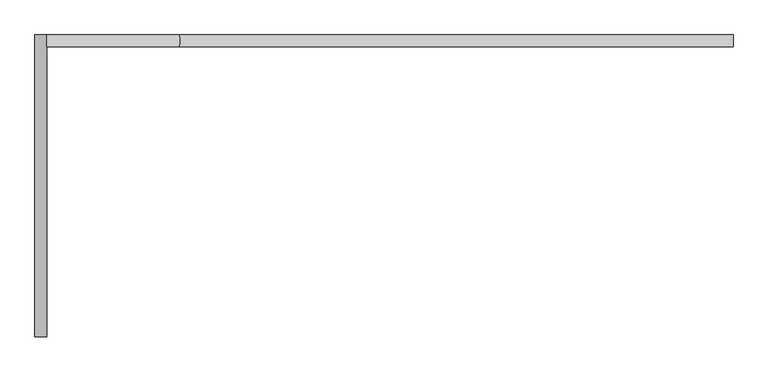
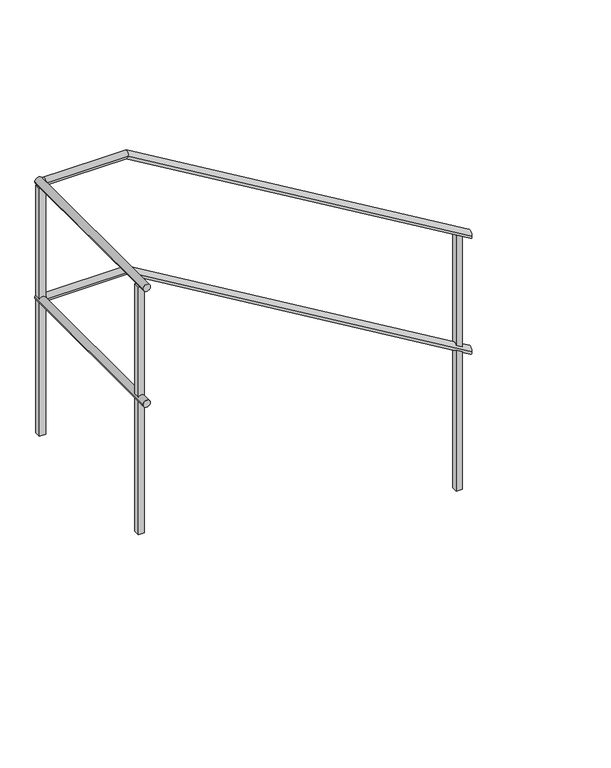
"""IFC4 building model written with IfcOpenShell, lengths in millimetres: railing geometry."""

from ifc_helpers import new_model, si_unit, frame, origin, place, context, project, spatial, polyline, circle_curve, ellipse_curve, outline, extrude, source, transform, mapped, element, save
from ifc_brep_helpers import plane_surface, cylinder_surface, advanced_brep


def railing_e85a09c7(model_context):
    return source(origin(), model_context, "Body", "SolidModel", [
        advanced_brep(
        [(33043.8956602, 24484.5208589, 749.1723166), (33043.8956602, 24514.5208589, 749.1723166), (31639.7692216, 24484.5208589, 1584.9618634), (31639.7692216, 24514.5208589, 1584.9618634), (31305.4, 24484.5208589, 1584.9618634), (31305.4, 24514.5208589, 1584.9618634)],
        [
            (0, 1, ellipse_curve(frame((33043.8956602, 24499.5208589, 749.1723166), z_axis=(1.0, 0.0, 0.0), x_axis=(0.0, 0.0, -1.0)), 17.4562134, 15.0)),
            (1, 0, ellipse_curve(frame((33043.8956602, 24499.5208589, 749.1723166), z_axis=(1.0, 0.0, 0.0), x_axis=(0.0, 0.0, -1.0)), 17.4562134, 15.0)),
            (0, 2),
            (2, 3, ellipse_curve(frame((31639.7692216, 24499.5208589, 1584.9618634), z_axis=(0.9641817474962141, 0.0, -0.2652424509673118), x_axis=(-0.265242450967312, 0.0, -0.9641817474962139)), 15.5572329, 15.0)),
            (3, 1),
            (3, 2, ellipse_curve(frame((31639.7692216, 24499.5208589, 1584.9618634), z_axis=(0.9641817474962141, 0.0, -0.2652424509673118), x_axis=(-0.265242450967312, 0.0, -0.9641817474962139)), 15.5572329, 15.0)),
            (4, 5, circle_curve(frame((31305.4, 24499.5208589, 1584.9618634), z_axis=(-1.0, 0.0, 0.0), x_axis=(0.0, 1.0, 0.0)), 15.0)),
            (5, 4, circle_curve(frame((31305.4, 24499.5208589, 1584.9618634), z_axis=(-1.0, 0.0, 0.0), x_axis=(0.0, 1.0, 0.0)), 15.0)),
            (2, 4),
            (5, 3),
        ],
        [
            plane_surface(frame((33043.8956602, 24499.5208589, 766.62853), z_axis=(1.0, 0.0, 0.0), x_axis=(0.0, -1.0, 0.0))),
            cylinder_surface(frame((33036.2234023, 24499.5208589, 753.7391368), z_axis=(0.8592928844097064, 0.0, -0.5114838597676831), x_axis=(0.0, 1.0, 0.0)), 15.0),
            plane_surface(frame((31305.4, 24499.5208589, 1599.9618634), z_axis=(-1.0, 0.0, 0.0), x_axis=(0.0, -1.0, 0.0))),
            cylinder_surface(frame((31643.8956602, 24499.5208589, 1584.9618634), z_axis=(1.0, 0.0, 0.0), x_axis=(0.0, 1.0, 0.0)), 15.0),
        ],
        [
            (0, [[1, 2]]),
            (1, [[-1, 3, 4, 5]]),
            (1, [[-2, -5, 6, -3]]),
            (2, [[7, 8]]),
            (3, [[-4, 9, -8, 10]]),
            (3, [[-6, -10, -7, -9]]),
        ],
    ),
        advanced_brep(
        [(33043.8956602, 24484.5208589, 1249.1723166), (33043.8956602, 24514.5208589, 1249.1723166), (31639.7692216, 24484.5208589, 2084.9618634), (31639.7692216, 24514.5208589, 2084.9618634), (31305.4, 24484.5208589, 2084.9618634), (31305.4, 24514.5208589, 2084.9618634)],
        [
            (0, 1, ellipse_curve(frame((33043.8956602, 24499.5208589, 1249.1723166), z_axis=(1.0, 0.0, 0.0), x_axis=(0.0, 0.0, -1.0)), 17.4562134, 15.0)),
            (1, 0, ellipse_curve(frame((33043.8956602, 24499.5208589, 1249.1723166), z_axis=(1.0, 0.0, 0.0), x_axis=(0.0, 0.0, -1.0)), 17.4562134, 15.0)),
            (0, 2),
            (2, 3, ellipse_curve(frame((31639.7692216, 24499.5208589, 2084.9618634), z_axis=(0.9641817474962141, 0.0, -0.2652424509673118), x_axis=(-0.265242450967312, 0.0, -0.9641817474962139)), 15.5572329, 15.0)),
            (3, 1),
            (3, 2, ellipse_curve(frame((31639.7692216, 24499.5208589, 2084.9618634), z_axis=(0.9641817474962141, 0.0, -0.2652424509673118), x_axis=(-0.265242450967312, 0.0, -0.9641817474962139)), 15.5572329, 15.0)),
            (4, 5, circle_curve(frame((31305.4, 24499.5208589, 2084.9618634), z_axis=(-1.0, 0.0, 0.0), x_axis=(0.0, 1.0, 0.0)), 15.0)),
            (5, 4, circle_curve(frame((31305.4, 24499.5208589, 2084.9618634), z_axis=(-1.0, 0.0, 0.0), x_axis=(0.0, 1.0, 0.0)), 15.0)),
            (2, 4),
            (5, 3),
        ],
        [
            plane_surface(frame((33043.8956602, 24499.5208589, 1266.62853), z_axis=(1.0, 0.0, 0.0), x_axis=(0.0, -1.0, 0.0))),
            cylinder_surface(frame((33036.2234023, 24499.5208589, 1253.7391368), z_axis=(0.8592928844097064, 0.0, -0.5114838597676831), x_axis=(0.0, 1.0, 0.0)), 15.0),
            plane_surface(frame((31305.4, 24499.5208589, 2099.9618634), z_axis=(-1.0, 0.0, 0.0), x_axis=(0.0, -1.0, 0.0))),
            cylinder_surface(frame((31643.8956602, 24499.5208589, 2084.9618634), z_axis=(1.0, 0.0, 0.0), x_axis=(0.0, 1.0, 0.0)), 15.0),
        ],
        [
            (0, [[1, 2]]),
            (1, [[-1, 3, 4, 5]]),
            (1, [[-2, -5, 6, -3]]),
            (2, [[7, 8]]),
            (3, [[-4, 9, -8, 10]]),
            (3, [[-6, -10, -7, -9]]),
        ],
    ),
        advanced_brep(
        [(31305.4, 24514.5208589, 1584.9618634), (31275.4, 24514.5208589, 1584.9618634), (31305.4, 23749.5208589, 1584.9618634), (31275.4, 23749.5208589, 1584.9618634)],
        [
            (0, 1, circle_curve(frame((31290.4, 24514.5208589, 1584.9618634), z_axis=(0.0, 1.0, 0.0), x_axis=(-1.0, 0.0, 0.0)), 15.0)),
            (1, 0, circle_curve(frame((31290.4, 24514.5208589, 1584.9618634), z_axis=(0.0, 1.0, 0.0), x_axis=(-1.0, 0.0, 0.0)), 15.0)),
            (2, 3, circle_curve(frame((31290.4, 23749.5208589, 1584.9618634), z_axis=(0.0, -1.0, 0.0), x_axis=(-1.0, 0.0, 0.0)), 15.0)),
            (3, 2, circle_curve(frame((31290.4, 23749.5208589, 1584.9618634), z_axis=(0.0, -1.0, 0.0), x_axis=(-1.0, 0.0, 0.0)), 15.0)),
            (0, 2),
            (3, 1),
        ],
        [
            plane_surface(frame((31290.4, 24514.5208589, 1599.9618634), z_axis=(0.0, 1.0, 0.0), x_axis=(0.0, 0.0, -1.0))),
            plane_surface(frame((31290.4, 23749.5208589, 1599.9618634), z_axis=(0.0, -1.0, 0.0), x_axis=(0.0, 0.0, -1.0))),
            cylinder_surface(frame((31290.4, 24514.5208589, 1584.9618634), z_axis=(0.0, 1.0, 0.0), x_axis=(-1.0, 0.0, 0.0)), 15.0),
        ],
        [
            (0, [[1, 2]]),
            (1, [[3, 4]]),
            (2, [[-1, 5, -4, 6]]),
            (2, [[-2, -6, -3, -5]]),
        ],
    ),
        advanced_brep(
        [(31305.4, 24514.5208589, 2084.9618634), (31275.4, 24514.5208589, 2084.9618634), (31305.4, 23749.5208589, 2084.9618634), (31275.4, 23749.5208589, 2084.9618634)],
        [
            (0, 1, circle_curve(frame((31290.4, 24514.5208589, 2084.9618634), z_axis=(0.0, 1.0, 0.0), x_axis=(-1.0, 0.0, 0.0)), 15.0)),
            (1, 0, circle_curve(frame((31290.4, 24514.5208589, 2084.9618634), z_axis=(0.0, 1.0, 0.0), x_axis=(-1.0, 0.0, 0.0)), 15.0)),
            (2, 3, circle_curve(frame((31290.4, 23749.5208589, 2084.9618634), z_axis=(0.0, -1.0, 0.0), x_axis=(-1.0, 0.0, 0.0)), 15.0)),
            (3, 2, circle_curve(frame((31290.4, 23749.5208589, 2084.9618634), z_axis=(0.0, -1.0, 0.0), x_axis=(-1.0, 0.0, 0.0)), 15.0)),
            (0, 2),
            (3, 1),
        ],
        [
            plane_surface(frame((31290.4, 24514.5208589, 2099.9618634), z_axis=(0.0, 1.0, 0.0), x_axis=(0.0, 0.0, -1.0))),
            plane_surface(frame((31290.4, 23749.5208589, 2099.9618634), z_axis=(0.0, -1.0, 0.0), x_axis=(0.0, 0.0, -1.0))),
            cylinder_surface(frame((31290.4, 24514.5208589, 2084.9618634), z_axis=(0.0, 1.0, 0.0), x_axis=(-1.0, 0.0, 0.0)), 15.0),
        ],
        [
            (0, [[1, 2]]),
            (1, [[3, 4]]),
            (2, [[-1, 5, -4, 6]]),
            (2, [[-2, -6, -3, -5]]),
        ],
    ),
        extrude(outline(polyline([(31302.9, 24512.0208589), (31302.9, 24487.0208589), (31277.9, 24487.0208589), (31277.9, 24512.0208589), (31302.9, 24512.0208589)])), frame((0.0, 0.0, 999.9618634), z_axis=(0.0, 0.0, 1.0), x_axis=(1.0, 0.0, 0.0)), (0.0, 0.0, 1.0), 1070.0),
        extrude(outline(polyline([(31277.9, 23812.0208589), (31302.9, 23812.0208589), (31302.9, 23787.0208589), (31277.9, 23787.0208589), (31277.9, 23812.0208589)])), frame((0.0, 0.0, 999.9618634), z_axis=(0.0, 0.0, 1.0), x_axis=(1.0, 0.0, 0.0)), (0.0, 0.0, 1.0), 1070.0),
        extrude(outline(polyline([(166.62853, 33006.3956602), (1258.9499586, 33006.3956602), (1273.830911, 32981.3956602), (166.62853, 32981.3956602), (166.62853, 33006.3956602)])), frame((0.0, 24487.0208589, 0.0), z_axis=(0.0, 1.0, 0.0), x_axis=(0.0, 0.0, 1.0)), (0.0, 0.0, 1.0), 25.0),
    ])


if __name__ == "__main__":
    model = new_model("IFC4")
    model_context = context("Model", 3, world=origin())
    ifc_project = project(units=[si_unit("LENGTHUNIT", "METRE", prefix="MILLI")], contexts=[model_context])
    site = spatial("IfcSite", under=ifc_project)
    building = spatial("IfcBuilding", under=site)
    placement = place(None, origin())
    railing_shape = railing_e85a09c7(model_context)
    element("IfcRailing", 1, at=placement, inside=building, context=model_context, shape_type="MappedRepresentation", body=[
        mapped(railing_shape, transform((0.0, 0.0, 0.0), x_axis=(1.0, 0.0, 0.0), y_axis=(0.0, 1.0, 0.0), z_axis=(0.0, 0.0, 1.0))),
    ])
    save(model, "model.ifc")
